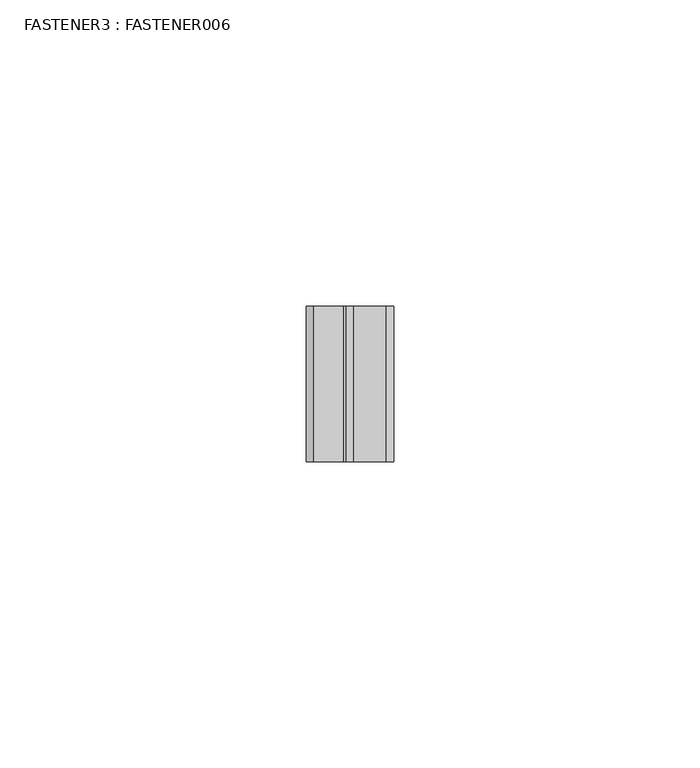
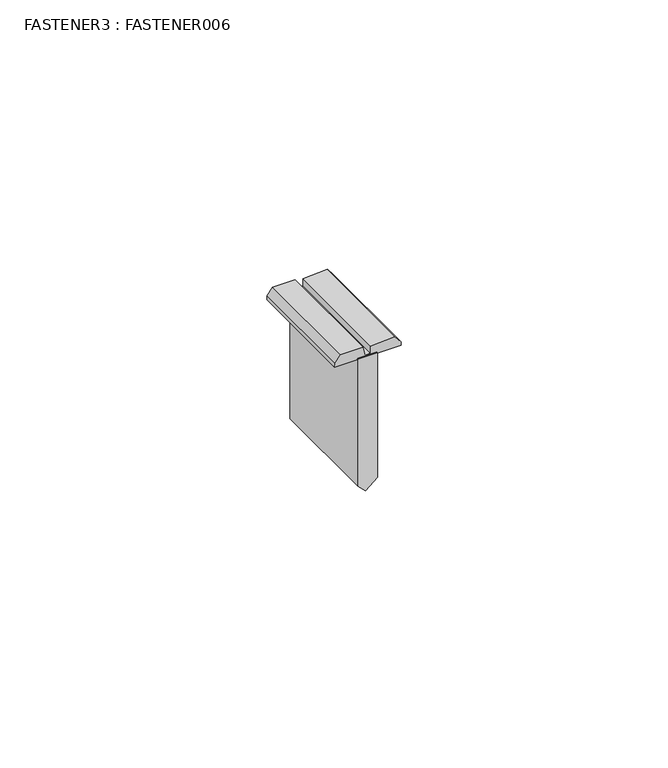
"""IFC4 building model written with IfcOpenShell, lengths in millimetres: proxy geometry, FASTENER3 : FASTENER006."""

from ifc_helpers import new_model, si_unit, frame, origin, place, context, project, spatial, polyline, outline, extrude, source, transform, mapped, element, save


def fastener3_fastener006_f031ca55(model_context):
    return source(origin(), model_context, "Body", "SweptSolid", [
        extrude(outline(polyline([(42577.1576024, 5870.6890035), (42548.1988623, 5870.6890035), (42546.5833096, 5872.3460181), (42548.7638676, 5874.895922), (42577.1576024, 5874.895922), (42577.1576024, 5870.6890035)])), frame((0.0, -1078.2906574, 0.0), z_axis=(0.0, 1.0, 0.0), x_axis=(0.0, 0.0, 1.0)), (0.0, 0.0, 1.0), 25.4),
        extrude(outline(polyline([(42577.1576024, 5879.9417891), (42577.9674245, 5879.9417891), (42579.5612959, 5878.7030871), (42579.1650604, 5873.4174049), (42577.5756297, 5873.4174049), (42577.5756297, 5872.1703), (42579.587761, 5871.7740645), (42579.587761, 5866.8949826), (42577.9938896, 5865.6562805), (42577.1576024, 5865.6454839), (42577.1576024, 5879.9417891)])), frame((0.0, -1078.2906574, 0.0), z_axis=(0.0, 1.0, 0.0), x_axis=(0.0, 0.0, 1.0)), (0.0, 0.0, 1.0), 25.4),
    ])


if __name__ == "__main__":
    model = new_model("IFC4")
    model_context = context("Model", 3, world=origin())
    ifc_project = project(units=[si_unit("LENGTHUNIT", "METRE", prefix="MILLI")], contexts=[model_context])
    site = spatial("IfcSite", under=ifc_project)
    building = spatial("IfcBuilding", under=site)
    placement = place(None, origin())
    fastener3_fastener006_shape = fastener3_fastener006_f031ca55(model_context)
    element("IfcBuildingElementProxy", 1, Name="FASTENER3 : FASTENER006", ObjectType="FASTENER3 : FASTENER006", at=placement, inside=building, context=model_context, shape_type="MappedRepresentation", body=[
        mapped(fastener3_fastener006_shape, transform((0.0, 0.0, 0.0), x_axis=(1.0, 0.0, 0.0), y_axis=(0.0, 1.0, 0.0), z_axis=(0.0, 0.0, 1.0))),
    ])
    save(model, "model.ifc")

# Revit data of these elements
# Type "FASTENER3 : FASTENER006"
#   NameOverride = "FASTENER006"
# Element 1 (IfcBuildingElementProxy, "FASTENER3 : FASTENER006")
#   Materials on its faces: "ENGINEERED PANCAKE HEAD FASTENER (NOT BY AEP-SPAN) @ 12\" O.C."
# Materials
#   "ENGINEERED PANCAKE HEAD FASTENER (NOT BY AEP-SPAN) @ 12\" O.C.": class "Unassigned", colour RGB 255 255 255, transparency 0
